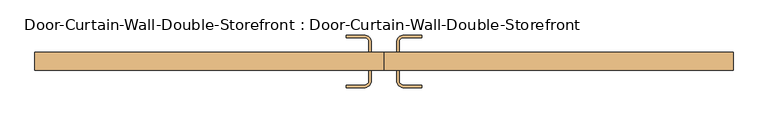
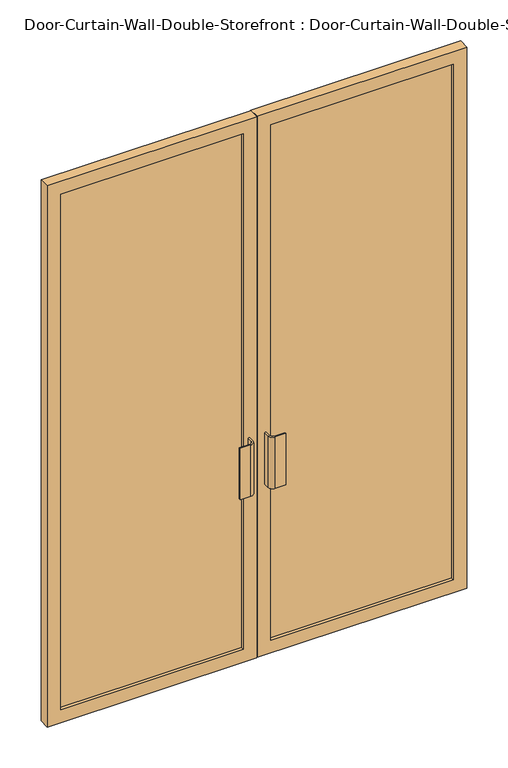
"""IFC4 building model written with IfcOpenShell, lengths in millimetres: door geometry, Door-Curtain-Wall-Double-Storefront : Door-Curtain-Wall-Double-Storefront."""

from ifc_helpers import new_model, si_unit, point, frame, frame_2d, origin, place, context, project, spatial, polyline, circle_curve, trimmed, segment, composite_curve, outline, extrude, source, transform, mapped, element, save


def door_curtain_wall_double_storefront_door_curtain_wall_double_9343b353(model_context):
    return source(origin(), model_context, "Body", "SweptSolid", [
        extrude(outline(polyline([(2406.65, 0.7668501), (0.0, 0.7668501), (0.0, 882.65), (2406.65, 882.65), (2406.65, 0.7668501)]), holes=[polyline([(2349.5, 57.9168501), (2349.5, 825.5), (57.15, 825.5), (57.15, 57.9168501), (2349.5, 57.9168501)])]), frame((0.0, -57.15, 0.0), z_axis=(0.0, 1.0, 0.0), x_axis=(0.0, 0.0, 1.0)), (0.0, 0.0, 1.0), 44.45),
        extrude(outline(polyline([(2406.65, -0.8206499), (2406.65, -882.65), (0.0, -882.65), (0.0, -0.8206499), (2406.65, -0.8206499)]), holes=[polyline([(2349.5, -825.5), (2349.5, -57.9706499), (57.15, -57.9706499), (57.15, -825.5), (2349.5, -825.5)])]), frame((0.0, -57.15, 0.0), z_axis=(0.0, 1.0, 0.0), x_axis=(0.0, 0.0, 1.0)), (0.0, 0.0, 1.0), 44.45),
        extrude(outline(polyline([(825.5, -25.4), (825.5, -44.45), (57.9168501, -44.45), (57.9168501, -25.4), (825.5, -25.4)])), frame((0.0, 0.0, 57.15), z_axis=(0.0, 0.0, 1.0), x_axis=(1.0, 0.0, 0.0)), (0.0, 0.0, 1.0), 2292.35),
        extrude(outline(polyline([(-57.9706499, -25.4), (-57.9706499, -44.45), (-825.5, -44.45), (-825.5, -25.4), (-57.9706499, -25.4)])), frame((0.0, 0.0, 57.15), z_axis=(0.0, 0.0, 1.0), x_axis=(1.0, 0.0, 0.0)), (0.0, 0.0, 1.0), 2292.35),
        extrude(outline(composite_curve([segment(polyline([(-31.7768999, 12.7), (-31.7768999, -12.7), (-38.1268999, -12.7), (-38.1268999, 12.7)]), True, "CONTINUOUS"), segment(trimmed(circle_curve(frame_2d((-50.8268999, 12.7)), 12.7), [point((-38.1268999, 12.7))], [point((-50.8268999, 25.4))], True, "CARTESIAN"), True, "CONTINUOUS"), segment(polyline([(-50.8268999, 25.4), (-95.2768999, 25.4), (-95.2768999, 31.75), (-50.8268999, 31.75)]), True, "CONTINUOUS"), segment(trimmed(circle_curve(frame_2d((-50.8268999, 12.7)), 19.05), [point((-50.8268999, 31.75))], [point((-31.7768999, 12.7))], False, "CARTESIAN"), True, "CONTINUOUS")], self_intersect=False)), frame((0.0, 0.0, 762.0), z_axis=(0.0, 0.0, 1.0), x_axis=(1.0, 0.0, 0.0)), (0.0, 0.0, 1.0), 228.6),
        extrude(outline(composite_curve([segment(trimmed(circle_curve(frame_2d((50.7731001, 12.7)), 19.05), [point((31.7231001, 12.7))], [point((50.7731001, 31.75))], False, "CARTESIAN"), True, "CONTINUOUS"), segment(polyline([(50.7731001, 31.75), (95.2231001, 31.75), (95.2231001, 25.4), (50.7731001, 25.4)]), True, "CONTINUOUS"), segment(trimmed(circle_curve(frame_2d((50.7731001, 12.7)), 12.7), [point((50.7731001, 25.4))], [point((38.0731001, 12.7))], True, "CARTESIAN"), True, "CONTINUOUS"), segment(polyline([(38.0731001, 12.7), (38.0731001, -12.7), (31.7231001, -12.7), (31.7231001, 12.7)]), True, "CONTINUOUS")], self_intersect=False)), frame((0.0, 0.0, 762.0), z_axis=(0.0, 0.0, 1.0), x_axis=(1.0, 0.0, 0.0)), (0.0, 0.0, 1.0), 228.6),
        extrude(outline(composite_curve([segment(trimmed(circle_curve(frame_2d((-50.8268999, -82.55)), 19.05), [point((-31.7768999, -82.55))], [point((-50.8268999, -101.6))], False, "CARTESIAN"), True, "CONTINUOUS"), segment(polyline([(-50.8268999, -101.6), (-95.2768999, -101.6), (-95.2768999, -95.25), (-50.8268999, -95.25)]), True, "CONTINUOUS"), segment(trimmed(circle_curve(frame_2d((-50.8268999, -82.55)), 12.7), [point((-50.8268999, -95.25))], [point((-38.1268999, -82.55))], True, "CARTESIAN"), True, "CONTINUOUS"), segment(polyline([(-38.1268999, -82.55), (-38.1268999, -57.15), (-31.7768999, -57.15), (-31.7768999, -82.55)]), True, "CONTINUOUS")], self_intersect=False)), frame((0.0, 0.0, 762.0), z_axis=(0.0, 0.0, 1.0), x_axis=(1.0, 0.0, 0.0)), (0.0, 0.0, 1.0), 228.6),
        extrude(outline(composite_curve([segment(polyline([(31.7231001, -82.55), (31.7231001, -57.15), (38.0731001, -57.15), (38.0731001, -82.55)]), True, "CONTINUOUS"), segment(trimmed(circle_curve(frame_2d((50.7731001, -82.55)), 12.7), [point((38.0731001, -82.55))], [point((50.7731001, -95.25))], True, "CARTESIAN"), True, "CONTINUOUS"), segment(polyline([(50.7731001, -95.25), (95.2231001, -95.25), (95.2231001, -101.6), (50.7731001, -101.6)]), True, "CONTINUOUS"), segment(trimmed(circle_curve(frame_2d((50.7731001, -82.55)), 19.05), [point((50.7731001, -101.6))], [point((31.7231001, -82.55))], False, "CARTESIAN"), True, "CONTINUOUS")], self_intersect=False)), frame((0.0, 0.0, 762.0), z_axis=(0.0, 0.0, 1.0), x_axis=(1.0, 0.0, 0.0)), (0.0, 0.0, 1.0), 228.6),
    ])


if __name__ == "__main__":
    model = new_model("IFC4")
    model_context = context("Model", 3, world=origin())
    ifc_project = project(units=[si_unit("LENGTHUNIT", "METRE", prefix="MILLI")], contexts=[model_context])
    site = spatial("IfcSite", under=ifc_project)
    building = spatial("IfcBuilding", under=site)
    placement = place(None, origin())
    door_curtain_wall_double_storefront_door_curtain_wall_double_shape = door_curtain_wall_double_storefront_door_curtain_wall_double_9343b353(model_context)
    element("IfcDoor", 1, ObjectType="Door-Curtain-Wall-Double-Storefront : Door-Curtain-Wall-Double-Storefront", at=placement, inside=building, context=model_context, shape_type="MappedRepresentation", body=[
        mapped(door_curtain_wall_double_storefront_door_curtain_wall_double_shape, transform((0.0, 0.0, 0.0), x_axis=(1.0, 0.0, 0.0), y_axis=(0.0, 1.0, 0.0), z_axis=(0.0, 0.0, 1.0))),
    ])
    save(model, "model.ifc")

# Revit data of these elements
# Type "Door-Curtain-Wall-Double-Storefront : Door-Curtain-Wall-Double-Storefront"
#   Type Mark = "17"
#   Construction Type Id = "opn-d46"
#   Assembly Code = "B2030100"
#   Analytic Construction = "Metal frame, double glass door"
#   Width [instance default] = 6' - 0"
#   Thermal Resistance (R) = 1.3794 (h·ft²·°F)/BTU
#   Swing Angle [instance default] = 90.00°
#   Panel Width [instance default] = 3' - 0"
#   Offset = 0' - 2 1/4"
#   Heat Transfer Coefficient (U) = 0.7250 BTU/(h·ft²·°F)
#   Define Thermal Properties by = 1
#   Function = 1
#   Frame Material = Aluminum
#   Door Handle Material = Aluminum
#   Glazing = Glass
#   Visual Light Transmittance = 0
#   Solar Heat Gain Coefficient = 0
# Element 1 (IfcDoor, "Door-Curtain-Wall-Double-Storefront : Door-Curtain-Wall-Double-Storefront")
#   Width = 5' - 9 1/2"
#   Panel Width = 2' - 10 3/4"
#   Materials on its faces: "Aluminum", "Glass"
# Materials
#   "Aluminum": class "Metal", colour RGB 247 247 247, transparency 0, Description = "Aluminum 6061", Cost = 0
#   "Glass": class "Glass", colour RGB 0 128 192, transparency 0.75, Description = "Soda Lime Glass", Cost = 0
